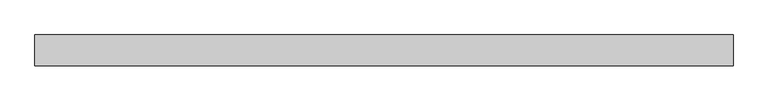
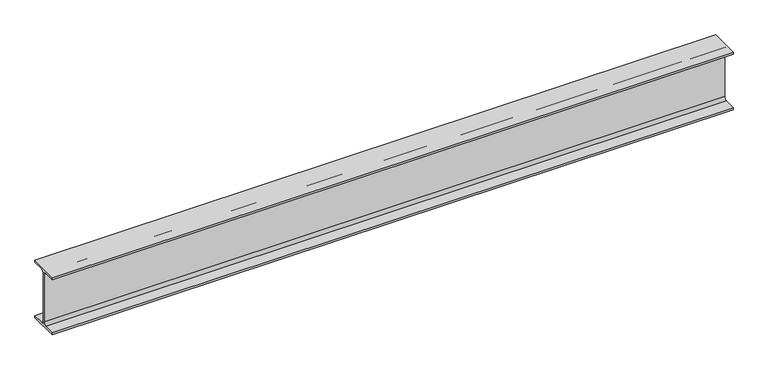
"""IFC4 building model written with IfcOpenShell, lengths in millimetres: beam geometry, 0912_Steel Framing_H-KSD3502 : H_SB_ASB_H-250x125x6x9."""

from ifc_helpers import new_model, si_unit, point, frame, frame_2d, origin, place, context, project, spatial, polyline, circle_curve, trimmed, segment, composite_curve, outline, extrude, source, transform, mapped, element, save


def beam_e570f850(model_context):
    return source(origin(), model_context, "Body", "SweptSolid", [
        extrude(outline(composite_curve([segment(polyline([(62.5, -116.0), (62.5, -125.0), (-62.5, -125.0), (-62.5, -116.0), (-15.0, -116.0)]), True, "CONTINUOUS"), segment(trimmed(circle_curve(frame_2d((-15.0, -104.0)), 12.0), [point((-15.0, -116.0))], [point((-3.0, -104.0))], True, "CARTESIAN"), True, "CONTINUOUS"), segment(polyline([(-3.0, -104.0), (-3.0, 104.0)]), True, "CONTINUOUS"), segment(trimmed(circle_curve(frame_2d((-15.0, 104.0)), 12.0), [point((-3.0, 104.0))], [point((-15.0, 116.0))], True, "CARTESIAN"), True, "CONTINUOUS"), segment(polyline([(-15.0, 116.0), (-62.5, 116.0), (-62.5, 125.0), (62.5, 125.0), (62.5, 116.0), (15.0, 116.0)]), True, "CONTINUOUS"), segment(trimmed(circle_curve(frame_2d((15.0, 104.0)), 12.0), [point((15.0, 116.0))], [point((3.0, 104.0))], True, "CARTESIAN"), True, "CONTINUOUS"), segment(polyline([(3.0, 104.0), (3.0, -104.0)]), True, "CONTINUOUS"), segment(trimmed(circle_curve(frame_2d((15.0, -104.0)), 12.0), [point((3.0, -104.0))], [point((15.0, -116.0))], True, "CARTESIAN"), True, "CONTINUOUS"), segment(polyline([(15.0, -116.0), (62.5, -116.0)]), True, "CONTINUOUS")], self_intersect=False)), frame((-1404.8000503, 0.0, 0.0), z_axis=(1.0, 0.0, 0.0), x_axis=(0.0, 1.0, 0.0)), (0.0, 0.0, 1.0), 2809.5192866),
    ])


if __name__ == "__main__":
    model = new_model("IFC4")
    model_context = context("Model", 3, world=origin())
    ifc_project = project(units=[si_unit("LENGTHUNIT", "METRE", prefix="MILLI")], contexts=[model_context])
    site = spatial("IfcSite", under=ifc_project)
    building = spatial("IfcBuilding", under=site)
    placement = place(None, origin())
    beam_shape = beam_e570f850(model_context)
    element("IfcBeam", 1, ObjectType="0912_Steel Framing_H-KSD3502 : H_SB_ASB_H-250x125x6x9", at=placement, inside=building, context=model_context, shape_type="MappedRepresentation", body=[
        mapped(beam_shape, transform((0.0, 0.0, 0.0), x_axis=(1.0, 0.0, 0.0), y_axis=(0.0, 1.0, 0.0), z_axis=(0.0, 0.0, 1.0))),
    ])
    save(model, "model.ifc")

# Revit data of these elements
# Type "0912_Steel Framing_H-KSD3502 : H_SB_ASB_H-250x125x6x9"
#   H_WM Code_1 = "S01AA003-00001 | Main Steel Structure Fabrication Work | Shelter/Building | Light Steel - Standard (30KG/M>Weight) | Material: (   )"
#   H_WM Code_2 = "S03AA029-00001 | Main Steel Structure Erection Work | Shelter/Building | Light Steel (30KG/M>Weight) | Material: (   )"
#   H_WM Code_3 = "S01AA010-00001 | Main Steel Structure Fabrication Work | Shelter/Building | Steel Painting/Coating | for Non-Fireproofed Steel Surface, Surface Preparation, Primer, Second & Final Coat | Material: (   )"
#   H_Q'ty Cal Type Tag = "SB-Q2"
#   Width = 12.5 cm
#   Web Thickness = 0.6 cm
#   Web Fillet = 1.2 cm
#   Warping Constant = 42539.8 cm⁶
#   W = 0
#   Torsional Moment of Inertia = 7.8102 cm⁴
#   Section Area = 37.66 cm²
#   Plastic Modulus weak axis = 73.1 cm³
#   Plastic Modulus strong axis = 366.0 cm³
#   Perimeter = 0.97 m²/m
#   Nominal Weight = 29.60 kgf/m
#   Moment of Inertia weak axis = 294.00 cm⁴
#   Moment of Inertia strong axis = 4050.00 cm⁴
#   Height = 25.0 cm
#   Flange Thickness = 0.9 cm
#   Elastic Modulus weak axis = 47.0 cm³
#   Elastic Modulus strong axis = 324.0 cm³
#   Centroid Vertical = 12.5 cm
#   Centroid Horizontal = 6.25 cm
#   Ix = 40500000
#   Length [instance default] = 1.5240 m
#   Zx = 366000
#   b = 0.1250 m
#   h = 0.2500 m
#   r = 0.0120 m
#   s = 0.0060 m
#   t = 0.0090 m
#   A = 0.003766 m²
#   Structural Material [instance default] = Steel, 45-345
#   Assembly Code = ""
# Element 1 (IfcBeam, "0912_Steel Framing_H-KSD3502 : H_SB_ASB_H-250x125x6x9")
#   Structural Material = none
# Materials
#   "Steel, 45-345": class "Metal", colour RGB 189 187 185, transparency 0, Description = "Steel 345 MPa", Cost = 0
